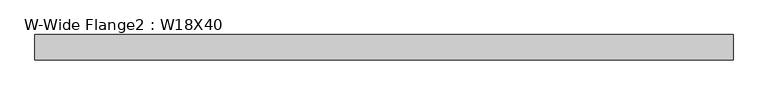
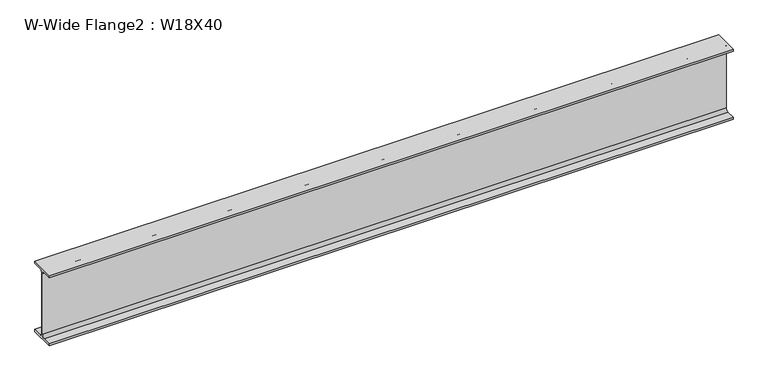
"""IFC4 building model written with IfcOpenShell, lengths in millimetres: beam geometry, W-Wide Flange2 : W18X40."""

from ifc_helpers import new_model, si_unit, point, frame, frame_2d, origin, place, context, project, spatial, polyline, circle_curve, trimmed, segment, composite_curve, outline, extrude, source, transform, mapped, element, save


def w_wide_flange2_w18x40_1003af5f(model_context):
    return source(origin(), model_context, "Body", "SweptSolid", [
        extrude(outline(composite_curve([segment(polyline([(76.454, -213.995), (76.454, -227.33), (-76.454, -227.33), (-76.454, -213.995), (-20.828, -213.995)]), True, "CONTINUOUS"), segment(trimmed(circle_curve(frame_2d((-20.828, -197.1675)), 16.8275), [point((-20.828, -213.995))], [point((-4.0005, -197.1675))], True, "CARTESIAN"), True, "CONTINUOUS"), segment(polyline([(-4.0005, -197.1675), (-4.0005, 197.1675)]), True, "CONTINUOUS"), segment(trimmed(circle_curve(frame_2d((-20.828, 197.1675)), 16.8275), [point((-4.0005, 197.1675))], [point((-20.828, 213.995))], True, "CARTESIAN"), True, "CONTINUOUS"), segment(polyline([(-20.828, 213.995), (-76.454, 213.995), (-76.454, 227.33), (76.454, 227.33), (76.454, 213.995), (20.828, 213.995)]), True, "CONTINUOUS"), segment(trimmed(circle_curve(frame_2d((20.828, 197.1675)), 16.8275), [point((20.828, 213.995))], [point((4.0005, 197.1675))], True, "CARTESIAN"), True, "CONTINUOUS"), segment(polyline([(4.0005, 197.1675), (4.0005, -197.1675)]), True, "CONTINUOUS"), segment(trimmed(circle_curve(frame_2d((20.828, -197.1675)), 16.8275), [point((4.0005, -197.1675))], [point((20.828, -213.995))], True, "CARTESIAN"), True, "CONTINUOUS"), segment(polyline([(20.828, -213.995), (76.454, -213.995)]), True, "CONTINUOUS")], self_intersect=False)), frame((-2095.246, 0.0, 0.0), z_axis=(1.0, 0.0, 0.0), x_axis=(0.0, 1.0, 0.0)), (0.0, 0.0, 1.0), 4190.492),
    ])


if __name__ == "__main__":
    model = new_model("IFC4")
    model_context = context("Model", 3, world=origin())
    ifc_project = project(units=[si_unit("LENGTHUNIT", "METRE", prefix="MILLI")], contexts=[model_context])
    site = spatial("IfcSite", under=ifc_project)
    building = spatial("IfcBuilding", under=site)
    placement = place(None, origin())
    w_wide_flange2_w18x40_shape = w_wide_flange2_w18x40_1003af5f(model_context)
    element("IfcBeam", 1, ObjectType="W-Wide Flange2 : W18X40", at=placement, inside=building, context=model_context, shape_type="MappedRepresentation", body=[
        mapped(w_wide_flange2_w18x40_shape, transform((0.0, 0.0, 0.0), x_axis=(1.0, 0.0, 0.0), y_axis=(0.0, 1.0, 0.0), z_axis=(0.0, 0.0, 1.0))),
    ])
    save(model, "model.ifc")

# Revit data of these elements
# Type "W-Wide Flange2 : W18X40"
#   Assembly Code = "B10"
#   W = 40
#   Length [instance default] = 5' - 0"
#   bf = 0' - 6.02"
#   d = 1' - 5.9"
#   k = 0' - 1 3/16"
#   k2 = 0' - 0.6625"
#   tf = 0' - 0.525"
#   tw = 0' - 0.315"
#   A = 0.0819444 SF
#   Structural Material [instance default] = Steel ASTM A992
# Element 1 (IfcBeam, "W-Wide Flange2 : W18X40")
#   Materials on its faces: "Steel ASTM A992"
# Materials
#   "Steel ASTM A992": class "Metal", colour RGB 199 199 199, transparency 0, Description = "Structural steel 50ksi", Cost = 0
